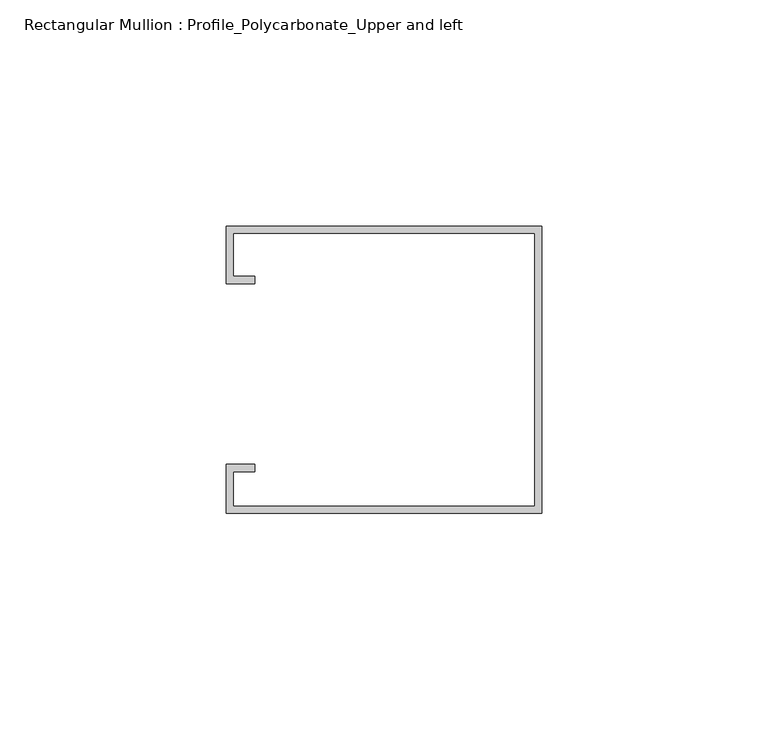
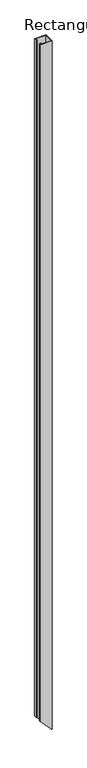
"""IFC4 building model written with IfcOpenShell, lengths in millimetres: member geometry, Rectangular Mullion : Profile_Polycarbonate_Upper and left."""

from ifc_helpers import new_model, si_unit, origin, place, context, project, spatial, faceted_brep, source, transform, mapped, element, save


def rectangular_mullion_profile_polycarbonate_upper_and_left_05964faa(model_context):
    return source(origin(), model_context, "Body", "Brep", [
        faceted_brep([(0.0, 32.7, 0.0), (-69.85, 32.7, 0.0), (-69.85, 20.0, 0.0), (-63.5, 20.0, 0.0), (-63.5, 21.5875, 0.0), (-68.2625, 21.5875, 0.0), (-68.2625, 31.1125, 0.0), (-1.5875, 31.1125, 0.0), (-1.5875, -29.2125, 0.0), (-68.2625, -29.2125, 0.0), (-68.2625, -21.5875, 0.0), (-63.5, -21.5875, 0.0), (-63.5, -20.0, 0.0), (-69.85, -20.0, 0.0), (-69.85, -30.8, 0.0), (0.0, -30.8, 0.0), (0.0, 32.7, -4472.3181431), (-69.85, 32.7, -4399.4971191), (-69.85, 20.0, -4399.4971191), (-63.5, 20.0, -4406.1172122), (-63.5, 21.5875, -4406.1172122), (-68.2625, 21.5875, -4401.1521423), (-68.2625, 31.1125, -4401.1521423), (-1.5875, 31.1125, -4470.6631198), (-1.5875, -29.2125, -4470.6631198), (-68.2625, -29.2125, -4401.1521423), (-68.2625, -21.5875, -4401.1521423), (-63.5, -21.5875, -4406.1172122), (-63.5, -20.0, -4406.1172122), (-69.85, -20.0, -4399.4971191), (-69.85, -30.8, -4399.4971191), (0.0, -30.8, -4472.3181431)], [[[0, 1, 2, 3, 4, 5, 6, 7, 8, 9, 10, 11, 12, 13, 14, 15]], [[1, 0, 16, 17]], [[2, 1, 17, 18]], [[3, 2, 18, 19]], [[4, 3, 19, 20]], [[5, 4, 20, 21]], [[6, 5, 21, 22]], [[7, 6, 22, 23]], [[8, 7, 23, 24]], [[9, 8, 24, 25]], [[10, 9, 25, 26]], [[11, 10, 26, 27]], [[12, 11, 27, 28]], [[13, 12, 28, 29]], [[14, 13, 29, 30]], [[15, 14, 30, 31]], [[0, 15, 31, 16]], [[16, 31, 30, 29, 28, 27, 26, 25, 24, 23, 22, 21, 20, 19, 18, 17]]]),
    ])


if __name__ == "__main__":
    model = new_model("IFC4")
    model_context = context("Model", 3, world=origin())
    ifc_project = project(units=[si_unit("LENGTHUNIT", "METRE", prefix="MILLI")], contexts=[model_context])
    site = spatial("IfcSite", under=ifc_project)
    building = spatial("IfcBuilding", under=site)
    placement = place(None, origin())
    rectangular_mullion_profile_polycarbonate_upper_and_left_shape = rectangular_mullion_profile_polycarbonate_upper_and_left_05964faa(model_context)
    element("IfcMember", 1, ObjectType="Rectangular Mullion : Profile_Polycarbonate_Upper and left", at=placement, inside=building, context=model_context, shape_type="MappedRepresentation", body=[
        mapped(rectangular_mullion_profile_polycarbonate_upper_and_left_shape, transform((0.0, 0.0, 0.0), x_axis=(1.0, 0.0, 0.0), y_axis=(0.0, 1.0, 0.0), z_axis=(0.0, 0.0, 1.0))),
    ])
    save(model, "model.ifc")

# Revit data of these elements
# Type "Rectangular Mullion : Profile_Polycarbonate_Upper and left"
#   built-in parameter 1007322 = 0.208333 (stored number, unit not read)
#   built-in parameter 1007321 = 0.00520833 (stored number, unit not read)
#   built-in parameter 1007320 = 0 (stored number, unit not read)
